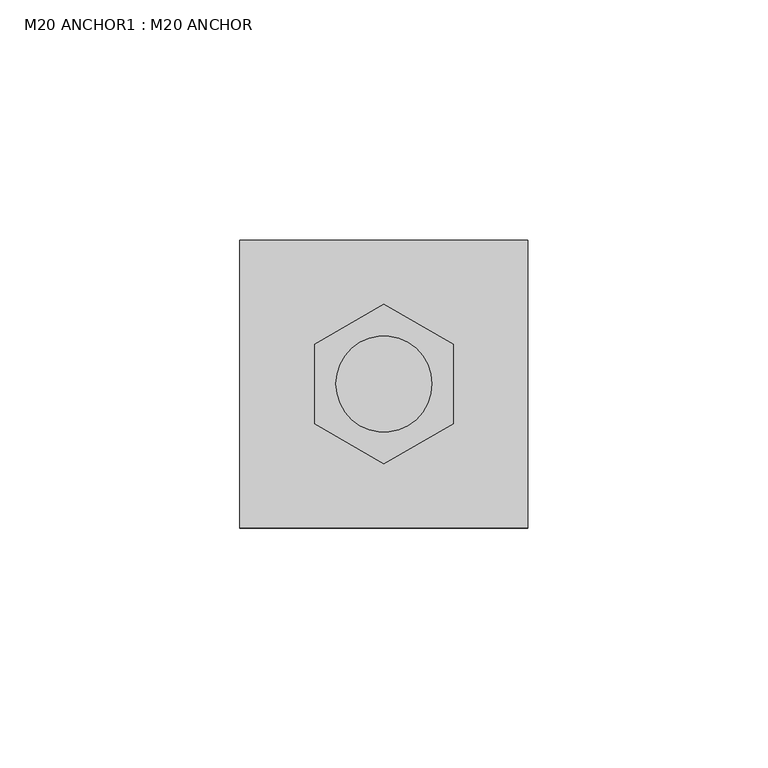
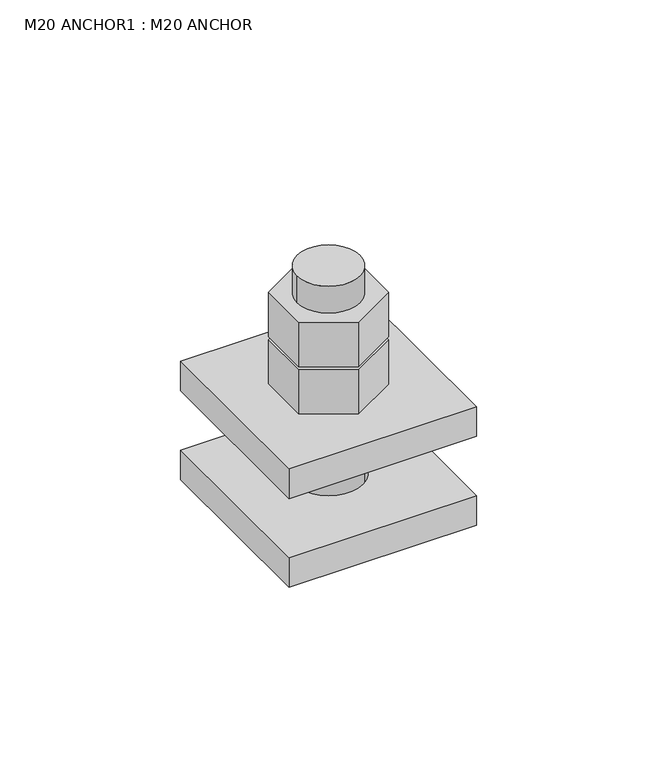
"""IFC4 building model written with IfcOpenShell, lengths in millimetres: fastener geometry, M20 ANCHOR1 : M20 ANCHOR."""

import ifcopenshell
import ifcopenshell.guid

model = None  # the IFC model being written
_history = None  # IfcOwnerHistory: only IFC2X3 demands one
_inside = {}  # id of a spatial element -> (the spatial element, [elements in it])
_under = {}  # id of a project, library or spatial element -> (it, [spatial elements below it])
_declared = {}  # id of a project -> (the project, [libraries it declares])
_typed = {}  # id of a type object -> (the type object, [elements of that type])
_made_of = {}  # id of a material, layer set ... -> (it, [elements and type objects made of it])


def new_model(schema):
    """Start an empty IFC model of exactly this schema.

    Asked for "IFC4X3", IfcOpenShell would pick the latest addendum, in which some entities
    have other attributes; the version numbers below select the first issue.
    IFC2X3 requires an IfcOwnerHistory on every rooted entity: one is made here for all.
    """
    global model, _history
    if schema == "IFC4X3":
        model = ifcopenshell.file(schema_version=(4, 3, 0, 0))
    else:
        model = ifcopenshell.file(schema=schema)
    _inside.clear()
    _under.clear()
    _declared.clear()
    _typed.clear()
    _made_of.clear()
    _history = None
    if model.schema == "IFC2X3":
        org = make("IfcOrganization", Name="unknown")
        user = make(
            "IfcPersonAndOrganization",
            ThePerson=make("IfcPerson", FamilyName="unknown"),
            TheOrganization=org,
        )
        app = make(
            "IfcApplication",
            ApplicationDeveloper=org,
            Version="unknown",
            ApplicationFullName="unknown",
            ApplicationIdentifier="unknown",
        )
        _history = make(
            "IfcOwnerHistory",
            OwningUser=user,
            OwningApplication=app,
            ChangeAction="ADDED",
            CreationDate=0,
        )
    return model


def make(cls, **values):
    """One entity of the class cls with the attributes given. An attribute that is None is left unset."""
    return model.create_entity(
        cls, **{name: value for name, value in values.items() if value is not None}
    )


def rooted(cls, **values):
    """An entity with a GlobalId (a new one), such as an element, a storey or a relation."""
    return make(cls, GlobalId=ifcopenshell.guid.new(), OwnerHistory=_history, **values)


def si_unit(unit_type, name, prefix=None):
    """IfcSIUnit, for example si_unit("LENGTHUNIT", "METRE", prefix="MILLI")."""
    return make("IfcSIUnit", UnitType=unit_type, Prefix=prefix, Name=name)


def assignment(units):
    """IfcUnitAssignment: the units of a project."""
    return None if units is None else make("IfcUnitAssignment", Units=units)


def point(xyz):
    """IfcCartesianPoint."""
    return None if xyz is None else make("IfcCartesianPoint", Coordinates=xyz)


def direction(xyz):
    """IfcDirection."""
    return None if xyz is None else make("IfcDirection", DirectionRatios=xyz)


def frame(location, z_axis=None, x_axis=None):
    """IfcAxis2Placement3D, a coordinate frame: its origin and axes. An axis left out is left unset."""
    return make(
        "IfcAxis2Placement3D",
        Location=point(location),
        Axis=direction(z_axis),
        RefDirection=direction(x_axis),
    )


def frame_2d(location, x_axis=None):
    """IfcAxis2Placement2D, a coordinate frame in the plane: its origin and x axis."""
    return make(
        "IfcAxis2Placement2D", Location=point(location), RefDirection=direction(x_axis)
    )


def origin():
    """The frame at (0, 0, 0) with its axes left unset."""
    return frame((0.0, 0.0, 0.0))


def place(relative_to, where):
    """IfcLocalPlacement: puts the frame where relative to a parent placement (None: the world)."""
    return make(
        "IfcLocalPlacement", PlacementRelTo=relative_to, RelativePlacement=where
    )


def context(
    kind, dimensions, precision=None, world=None, true_north=None, identifier=None
):
    """IfcGeometricRepresentationContext, for example the 3D "Model" context."""
    return make(
        "IfcGeometricRepresentationContext",
        ContextIdentifier=identifier,
        ContextType=kind,
        CoordinateSpaceDimension=dimensions,
        Precision=precision,
        WorldCoordinateSystem=world,
        TrueNorth=true_north,
    )


def project(units=None, contexts=None):
    """IfcProject with its units and contexts."""
    return rooted(
        "IfcProject",
        Name="project",
        RepresentationContexts=contexts,
        UnitsInContext=assignment(units),
    )


def spatial(cls, under=None, at=None, **own):
    """A site, building, storey or space (cls), placed at a placement, below another one or the project."""
    s = rooted(cls, ObjectPlacement=at, **own)
    if under is not None:
        _under.setdefault(under.id(), (under, []))[1].append(s)
    return s


def polyline(points):
    """IfcPolyline through the points."""
    return make("IfcPolyline", Points=[point(p) for p in points])


def circle_curve(where, radius):
    """IfcCircle in the frame where."""
    return make("IfcCircle", Position=where, Radius=radius)


def trimmed(basis, trim1, trim2, sense, master):
    """IfcTrimmedCurve: the piece of a basis curve between two trims."""
    return make(
        "IfcTrimmedCurve",
        BasisCurve=basis,
        Trim1=trim1,
        Trim2=trim2,
        SenseAgreement=sense,
        MasterRepresentation=master,
    )


def segment(curve, same_sense, transition):
    """IfcCompositeCurveSegment."""
    return make(
        "IfcCompositeCurveSegment",
        Transition=transition,
        SameSense=same_sense,
        ParentCurve=curve,
    )


def composite_curve(segments, self_intersect=None):
    """IfcCompositeCurve: segments joined end to end."""
    return make("IfcCompositeCurve", Segments=segments, SelfIntersect=self_intersect)


def outline(outer, holes=None, kind="AREA"):
    """IfcArbitraryClosedProfileDef: a profile drawn as a closed curve; with holes, ...WithVoids."""
    if holes is None:
        return make("IfcArbitraryClosedProfileDef", ProfileType=kind, OuterCurve=outer)
    return make(
        "IfcArbitraryProfileDefWithVoids",
        ProfileType=kind,
        OuterCurve=outer,
        InnerCurves=holes,
    )


def extrude(swept, where, along, depth):
    """IfcExtrudedAreaSolid: the profile swept, set in the frame where, extruded along a direction by depth."""
    return make(
        "IfcExtrudedAreaSolid",
        SweptArea=swept,
        Position=where,
        ExtrudedDirection=direction(along),
        Depth=depth,
    )


def shape(context_of_items, identifier, shape_type, items):
    """IfcShapeRepresentation: the items that make up one representation, for example the "Body"."""
    return make(
        "IfcShapeRepresentation",
        ContextOfItems=context_of_items,
        RepresentationIdentifier=identifier,
        RepresentationType=shape_type,
        Items=items,
    )


def source(mapping_origin, context_of_items, identifier, shape_type, items):
    """IfcRepresentationMap: a shape defined once, which mapped items show again and again."""
    return make(
        "IfcRepresentationMap",
        MappingOrigin=mapping_origin,
        MappedRepresentation=shape(context_of_items, identifier, shape_type, items),
    )


def transform(
    local_origin,
    x_axis=None,
    y_axis=None,
    z_axis=None,
    scale=None,
    scale2=None,
    scale3=None,
    uniform=True,
):
    """IfcCartesianTransformationOperator3D, or its non-uniform kind. x_axis, y_axis, z_axis: its Axis1, 2, 3."""
    if uniform:
        return make(
            "IfcCartesianTransformationOperator3D",
            Axis1=direction(x_axis),
            Axis2=direction(y_axis),
            LocalOrigin=point(local_origin),
            Scale=scale,
            Axis3=direction(z_axis),
        )
    return make(
        "IfcCartesianTransformationOperator3DnonUniform",
        Axis1=direction(x_axis),
        Axis2=direction(y_axis),
        LocalOrigin=point(local_origin),
        Scale=scale,
        Axis3=direction(z_axis),
        Scale2=scale2,
        Scale3=scale3,
    )


def mapped(mapping_source, mapping_target):
    """IfcMappedItem: shows the shape of a source again, moved by a transform."""
    return make(
        "IfcMappedItem", MappingSource=mapping_source, MappingTarget=mapping_target
    )


def made_of(thing, what):
    """Note that an element or type object is made of a material, layer set ...; save() writes the relation."""
    if what is not None:
        _made_of.setdefault(what.id(), (what, []))[1].append(thing)
    return thing


def element(
    cls,
    number,
    at=None,
    inside=None,
    cuts=None,
    type_object=None,
    material=None,
    context=None,
    identifier="Body",
    shape_type=None,
    held_by="IfcProductDefinitionShape",
    body=None,
    shapes=None,
    **own,
):
    """One element of the class cls, such as IfcWall. Its Tag is "e" and its number.

    at: its placement. inside: the storey or other place that contains it. cuts: it is an
    opening in that element (IfcRelVoidsElement). A single representation is given by context,
    identifier, shape_type and body (its items); several are given by shapes. held_by: the class
    of the entity that holds the representations. save() writes the other relations.
    """
    e = rooted(cls, Tag="e%d" % number, ObjectPlacement=at, **own)
    if body is not None:
        shapes = [shape(context, identifier, shape_type, body)]
    if shapes is not None:
        e.Representation = make(held_by, Representations=shapes)
    if inside is not None:
        _inside.setdefault(inside.id(), (inside, []))[1].append(e)
    if cuts is not None:
        rooted(
            "IfcRelVoidsElement", RelatingBuildingElement=cuts, RelatedOpeningElement=e
        )
    if type_object is not None:
        _typed.setdefault(type_object.id(), (type_object, []))[1].append(e)
    return made_of(e, material)


def aggregate(whole, parts):
    """IfcRelAggregates: a whole, such as a stair, and the parts it consists of."""
    return rooted("IfcRelAggregates", RelatingObject=whole, RelatedObjects=parts)


def save(model, path):
    """Write the relations noted so far, then the file.

    IfcRelAggregates (storeys below a building ...), IfcRelContainedInSpatialStructure (elements
    in a storey), IfcRelDefinesByType, IfcRelAssociatesMaterial and IfcRelDeclares: one each for
    every whole, place, type object, material and project.
    """
    for whole, parts in _under.values():
        aggregate(whole, parts)
    for where, things in _inside.values():
        rooted(
            "IfcRelContainedInSpatialStructure",
            RelatedElements=things,
            RelatingStructure=where,
        )
    for kind, things in _typed.values():
        rooted("IfcRelDefinesByType", RelatedObjects=things, RelatingType=kind)
    for what, things in _made_of.values():
        rooted("IfcRelAssociatesMaterial", RelatedObjects=things, RelatingMaterial=what)
    for by, libraries in _declared.values():
        rooted("IfcRelDeclares", RelatingContext=by, RelatedDefinitions=libraries)
    model.write(path)


def m20_anchor1_m20_anchor_b60c8576(model_context):
    return source(origin(), model_context, "Body", "SweptSolid", [
        extrude(outline(polyline([(-8.0855968, 19453.9464399), (-22.4937158, 19445.6279085), (-36.9018348, 19453.9464399), (-36.9018348, 19470.5835027), (-22.4937158, 19478.9020341), (-8.0855968, 19470.5835027), (-8.0855968, 19453.9464399)]), holes=[composite_curve([segment(trimmed(circle_curve(frame_2d((-22.4937158, 19462.2649713)), 10.0), [point((-32.4937158, 19462.2649713))], [point((-12.4937158, 19462.2649713))], True, "CARTESIAN"), True, "CONTINUOUS"), segment(trimmed(circle_curve(frame_2d((-22.4937158, 19462.2649713)), 10.0), [point((-12.4937158, 19462.2649713))], [point((-32.4937158, 19462.2649713))], True, "CARTESIAN"), True, "CONTINUOUS")], self_intersect=False)]), frame((0.0, 0.0, 246.0), z_axis=(0.0, 0.0, 1.0), x_axis=(1.0, 0.0, 0.0)), (0.0, 0.0, 1.0), 15.0),
        extrude(outline(polyline([(-8.0855968, 19453.9464399), (-22.4937158, 19445.6279085), (-36.9018348, 19453.9464399), (-36.9018348, 19470.5835027), (-22.4937158, 19478.9020341), (-8.0855968, 19470.5835027), (-8.0855968, 19453.9464399)]), holes=[composite_curve([segment(trimmed(circle_curve(frame_2d((-22.4937158, 19462.2649713)), 10.0), [point((-32.4937158, 19462.2649713))], [point((-12.4937158, 19462.2649713))], True, "CARTESIAN"), True, "CONTINUOUS"), segment(trimmed(circle_curve(frame_2d((-22.4937158, 19462.2649713)), 10.0), [point((-12.4937158, 19462.2649713))], [point((-32.4937158, 19462.2649713))], True, "CARTESIAN"), True, "CONTINUOUS")], self_intersect=False)]), frame((0.0, 0.0, 230.0), z_axis=(0.0, 0.0, 1.0), x_axis=(1.0, 0.0, 0.0)), (0.0, 0.0, 1.0), 15.0),
        extrude(outline(composite_curve([segment(trimmed(circle_curve(frame_2d((-22.4937158, 19462.2649713)), 10.0), [point((-32.4937158, 19462.2649713))], [point((-12.4937158, 19462.2649713))], False, "CARTESIAN"), True, "CONTINUOUS"), segment(trimmed(circle_curve(frame_2d((-22.4937158, 19462.2649713)), 10.0), [point((-12.4937158, 19462.2649713))], [point((-32.4937158, 19462.2649713))], False, "CARTESIAN"), True, "CONTINUOUS")], self_intersect=False)), frame((0.0, 0.0, 190.0), z_axis=(0.0, 0.0, 1.0), x_axis=(1.0, 0.0, 0.0)), (0.0, 0.0, 1.0), 80.0),
        extrude(outline(polyline([(7.5062842, 19432.2649713), (-52.4937158, 19432.2649713), (-52.4937158, 19492.2649713), (7.5062842, 19492.2649713), (7.5062842, 19432.2649713)]), holes=[composite_curve([segment(trimmed(circle_curve(frame_2d((-22.4937158, 19462.2649713)), 11.0), [point((-33.4937158, 19462.2649713))], [point((-11.4937158, 19462.2649713))], True, "CARTESIAN"), True, "CONTINUOUS"), segment(trimmed(circle_curve(frame_2d((-22.4937158, 19462.2649713)), 11.0), [point((-11.4937158, 19462.2649713))], [point((-33.4937158, 19462.2649713))], True, "CARTESIAN"), True, "CONTINUOUS")], self_intersect=False)]), frame((0.0, 0.0, 190.0), z_axis=(0.0, 0.0, 1.0), x_axis=(1.0, 0.0, 0.0)), (0.0, 0.0, 1.0), 10.0),
        extrude(outline(polyline([(7.5062842, 19432.2649713), (-52.4937158, 19432.2649713), (-52.4937158, 19492.2649713), (7.5062842, 19492.2649713), (7.5062842, 19432.2649713)]), holes=[composite_curve([segment(trimmed(circle_curve(frame_2d((-22.4937158, 19462.2649713)), 11.0), [point((-33.4937158, 19462.2649713))], [point((-11.4937158, 19462.2649713))], True, "CARTESIAN"), True, "CONTINUOUS"), segment(trimmed(circle_curve(frame_2d((-22.4937158, 19462.2649713)), 11.0), [point((-11.4937158, 19462.2649713))], [point((-33.4937158, 19462.2649713))], True, "CARTESIAN"), True, "CONTINUOUS")], self_intersect=False)]), frame((0.0, 0.0, 220.0), z_axis=(0.0, 0.0, 1.0), x_axis=(1.0, 0.0, 0.0)), (0.0, 0.0, 1.0), 10.0),
    ])


if __name__ == "__main__":
    model = new_model("IFC4")
    model_context = context("Model", 3, world=origin())
    ifc_project = project(units=[si_unit("LENGTHUNIT", "METRE", prefix="MILLI")], contexts=[model_context])
    site = spatial("IfcSite", under=ifc_project)
    building = spatial("IfcBuilding", under=site)
    placement = place(None, origin())
    m20_anchor1_m20_anchor_shape = m20_anchor1_m20_anchor_b60c8576(model_context)
    element("IfcFastener", 1, ObjectType="M20 ANCHOR1 : M20 ANCHOR", at=placement, inside=building, context=model_context, shape_type="MappedRepresentation", body=[
        mapped(m20_anchor1_m20_anchor_shape, transform((0.0, 0.0, 0.0), x_axis=(1.0, 0.0, 0.0), y_axis=(0.0, 1.0, 0.0), z_axis=(0.0, 0.0, 1.0))),
    ])
    save(model, "model.ifc")
